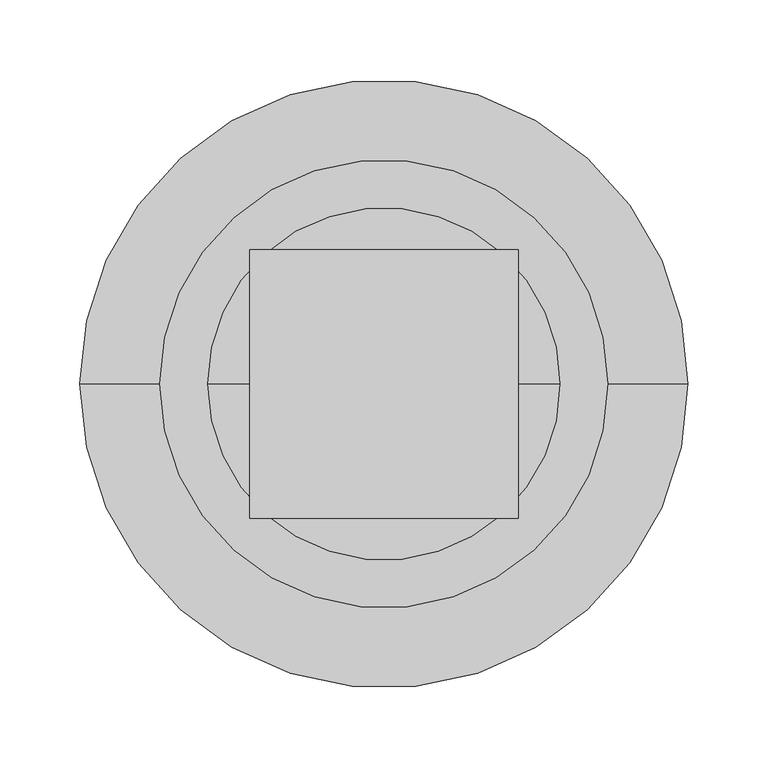
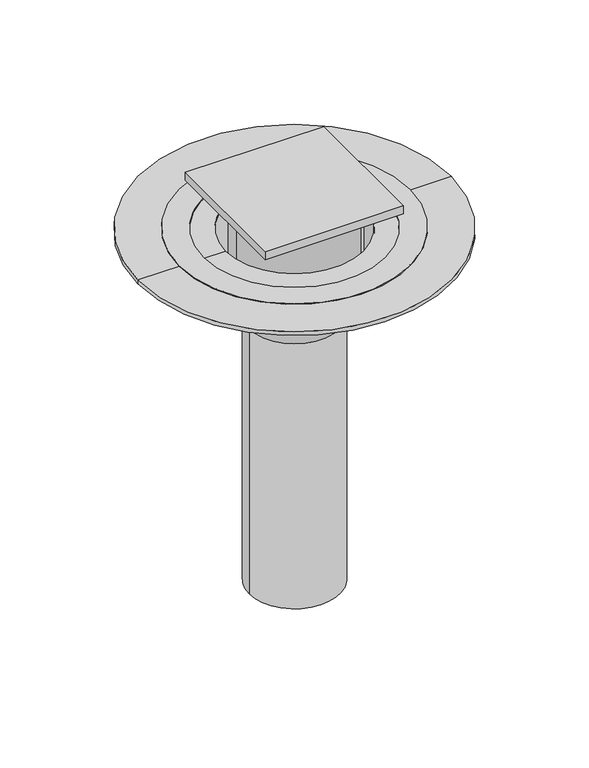
"""IFC4 building model written with IfcOpenShell, lengths in millimetres: proxy geometry, TN_Надставной элемент водоприемной воронки : Надставной элемент с обжимным закручивающемся фланцем, уплотнительным кольцом и трапом для эксплуатируемой кровли."""

from ifc_helpers import new_model, si_unit, point, frame, origin, origin_with_axes, origin_2d, place, context, project, spatial, polyline, circle_curve, trimmed, segment, composite_curve, outline, extrude, source, transform, mapped, element, save
from ifc_brep_helpers import plane_surface, cylinder_surface, revolved_surface, advanced_brep


def specialty_equipment_4cfdb0cb(model_context):
    return source(origin(), model_context, "Body", "SolidModel", [
        extrude(outline(composite_curve([segment(trimmed(circle_curve(origin_2d(), 70.0), [point((-70.0, 0.0))], [point((70.0, 0.0))], False, "CARTESIAN"), True, "CONTINUOUS"), segment(trimmed(circle_curve(origin_2d(), 70.0), [point((70.0, 0.0))], [point((-70.0, 0.0))], False, "CARTESIAN"), True, "CONTINUOUS")], self_intersect=False)), frame((0.0, 0.0, -66.9669914), z_axis=(0.0, 0.0, 1.0), x_axis=(1.0, 0.0, 0.0)), (0.0, 0.0, 1.0), 106.9669914),
        extrude(outline(polyline([(83.890873, 83.890873), (83.890873, -83.890873), (-83.890873, -83.890873), (-83.890873, 83.890873), (83.890873, 83.890873)])), frame((0.0, 0.0, 40.0), z_axis=(0.0, 0.0, 1.0), x_axis=(1.0, 0.0, 0.0)), (0.0, 0.0, 1.0), 10.0),
        extrude(outline(composite_curve([segment(trimmed(circle_curve(origin_2d(), 140.0), [point((-140.0, 0.0))], [point((140.0, 0.0))], False, "CARTESIAN"), True, "CONTINUOUS"), segment(trimmed(circle_curve(origin_2d(), 140.0), [point((140.0, 0.0))], [point((-140.0, 0.0))], False, "CARTESIAN"), True, "CONTINUOUS")], self_intersect=False), holes=[composite_curve([segment(trimmed(circle_curve(origin_2d(), 110.0556416), [point((-110.0556416, 0.0))], [point((110.0556416, 0.0))], True, "CARTESIAN"), True, "CONTINUOUS"), segment(trimmed(circle_curve(origin_2d(), 110.0556416), [point((110.0556416, 0.0))], [point((-110.0556416, 0.0))], True, "CARTESIAN"), True, "CONTINUOUS")], self_intersect=False)]), origin_with_axes(), (0.0, 0.0, 1.0), 1.0),
        advanced_brep(
        [(0.0, 0.0, -450.0), (-55.0, 0.0, -450.0), (55.0, 0.0, -450.0), (190.0, 0.0, 0.0), (-190.0, 0.0, 0.0), (-83.890873, 0.0, 0.0), (83.890873, 0.0, 0.0), (190.0, 0.0, -5.0), (-190.0, 0.0, -5.0), (93.890873, 0.0, -5.0), (-93.890873, 0.0, -5.0), (55.0, 0.0, -110.0), (-55.0, 0.0, -110.0), (-93.890873, 0.0, -71.109127), (93.890873, 0.0, -71.109127), (55.5025253, 0.0, -95.3553391), (-55.5025253, 0.0, -95.3553391), (0.0, 0.0, -95.3553391), (83.890873, 0.0, -66.9669914), (-83.890873, 0.0, -66.9669914)],
        [
            (0, 1),
            (1, 2, circle_curve(frame((0.0, 0.0, -450.0), z_axis=(0.0, 0.0, -1.0), x_axis=(-1.0, 0.0, 0.0)), 55.0)),
            (2, 0),
            (2, 1, circle_curve(frame((0.0, 0.0, -450.0), z_axis=(0.0, 0.0, -1.0), x_axis=(-1.0, 0.0, 0.0)), 55.0)),
            (3, 4, circle_curve(frame((0.0, 0.0, 0.0), z_axis=(0.0, 0.0, 1.0), x_axis=(-1.0, 0.0, 0.0)), 190.0)),
            (4, 5),
            (5, 6, circle_curve(frame((0.0, 0.0, 0.0), z_axis=(0.0, 0.0, -1.0), x_axis=(-1.0, 0.0, 0.0)), 83.890873)),
            (6, 3),
            (4, 3, circle_curve(frame((0.0, 0.0, 0.0), z_axis=(0.0, 0.0, 1.0), x_axis=(-1.0, 0.0, 0.0)), 190.0)),
            (6, 5, circle_curve(frame((0.0, 0.0, 0.0), z_axis=(0.0, 0.0, -1.0), x_axis=(-1.0, 0.0, 0.0)), 83.890873)),
            (7, 8, circle_curve(frame((0.0, 0.0, -5.0), z_axis=(0.0, 0.0, 1.0), x_axis=(-1.0, 0.0, 0.0)), 190.0)),
            (8, 4),
            (3, 7),
            (8, 7, circle_curve(frame((0.0, 0.0, -5.0), z_axis=(0.0, 0.0, 1.0), x_axis=(-1.0, 0.0, 0.0)), 190.0)),
            (9, 10, circle_curve(frame((0.0, 0.0, -5.0), z_axis=(0.0, 0.0, 1.0), x_axis=(-1.0, 0.0, 0.0)), 93.890873)),
            (10, 8),
            (7, 9),
            (10, 9, circle_curve(frame((0.0, 0.0, -5.0), z_axis=(0.0, 0.0, 1.0), x_axis=(-1.0, 0.0, 0.0)), 93.890873)),
            (11, 12, circle_curve(frame((0.0, 0.0, -110.0), z_axis=(0.0, 0.0, 1.0), x_axis=(-1.0, 0.0, 0.0)), 55.0)),
            (12, 13),
            (13, 14, circle_curve(frame((0.0, 0.0, -71.109127), z_axis=(0.0, 0.0, -1.0), x_axis=(-1.0, 0.0, 0.0)), 93.890873)),
            (14, 11),
            (12, 11, circle_curve(frame((0.0, 0.0, -110.0), z_axis=(0.0, 0.0, 1.0), x_axis=(-1.0, 0.0, 0.0)), 55.0)),
            (14, 13, circle_curve(frame((0.0, 0.0, -71.109127), z_axis=(0.0, 0.0, -1.0), x_axis=(-1.0, 0.0, 0.0)), 93.890873)),
            (1, 12),
            (11, 2),
            (13, 10),
            (9, 14),
            (15, 16, circle_curve(frame((0.0, 0.0, -95.3553391), z_axis=(0.0, 0.0, 1.0), x_axis=(-1.0, 0.0, 0.0)), 55.5025253)),
            (16, 17),
            (17, 15),
            (16, 15, circle_curve(frame((0.0, 0.0, -95.3553391), z_axis=(0.0, 0.0, 1.0), x_axis=(-1.0, 0.0, 0.0)), 55.5025253)),
            (18, 19, circle_curve(frame((0.0, 0.0, -66.9669914), z_axis=(0.0, 0.0, 1.0), x_axis=(-1.0, 0.0, 0.0)), 83.890873)),
            (19, 16),
            (15, 18),
            (19, 18, circle_curve(frame((0.0, 0.0, -66.9669914), z_axis=(0.0, 0.0, 1.0), x_axis=(-1.0, 0.0, 0.0)), 83.890873)),
            (5, 19),
            (18, 6),
        ],
        [
            plane_surface(frame((0.0, 0.0, -450.0), z_axis=(0.0, 0.0, -1.0), x_axis=(-1.0, 0.0, 0.0))),
            plane_surface(frame((0.0, 0.0, 0.0), z_axis=(0.0, 0.0, 1.0), x_axis=(-1.0, 0.0, 0.0))),
            cylinder_surface(frame((0.0, 0.0, 0.0), z_axis=(0.0, 0.0, -1.0), x_axis=(-1.0, 0.0, 0.0)), 190.0),
            plane_surface(frame((0.0, 0.0, -5.0), z_axis=(0.0, 0.0, -1.0), x_axis=(-1.0, 0.0, 0.0))),
            revolved_surface(polyline([(-93.890873, 0.0, -71.109127), (-55.0, 0.0, -110.0)]), (0.0, 0.0, 0.0), (0.0, 0.0, -1.0)),
            cylinder_surface(frame((0.0, 0.0, 0.0), z_axis=(0.0, 0.0, -1.0), x_axis=(-1.0, 0.0, 0.0)), 55.0),
            cylinder_surface(frame((0.0, 0.0, 0.0), z_axis=(0.0, 0.0, -1.0), x_axis=(-1.0, 0.0, 0.0)), 93.890873),
            plane_surface(frame((0.0, 0.0, -95.3553391), z_axis=(0.0, 0.0, 1.0), x_axis=(-1.0, 0.0, 0.0))),
            revolved_surface(polyline([(-55.5025253, 0.0, -95.3553391), (-83.890873, 0.0, -66.9669914)]), (0.0, 0.0, 0.0), (0.0, 0.0, -1.0)),
            revolved_surface(polyline([(-83.890873, 0.0, -66.9669914), (-83.890873, 0.0, 0.0)]), (0.0, 0.0, 0.0), (0.0, 0.0, -1.0)),
        ],
        [
            (0, [[1, 2, 3]]),
            (0, [[-3, 4, -1]]),
            (1, [[5, 6, 7, 8]]),
            (1, [[9, -8, 10, -6]]),
            (2, [[11, 12, -5, 13]]),
            (2, [[14, -13, -9, -12]]),
            (3, [[15, 16, -11, 17]]),
            (3, [[18, -17, -14, -16]]),
            (4, [[19, 20, 21, 22]]),
            (4, [[23, -22, 24, -20]]),
            (5, [[-2, 25, -19, 26]]),
            (5, [[-4, -26, -23, -25]]),
            (6, [[-21, 27, -15, 28]]),
            (6, [[-24, -28, -18, -27]]),
            (7, [[29, 30, 31]]),
            (7, [[32, -31, -30]]),
            (8, [[33, 34, -29, 35]]),
            (8, [[36, -35, -32, -34]]),
            (9, [[-7, 37, -33, 38]]),
            (9, [[-10, -38, -36, -37]]),
        ],
    ),
    ])


if __name__ == "__main__":
    model = new_model("IFC4")
    model_context = context("Model", 3, world=origin())
    ifc_project = project(units=[si_unit("LENGTHUNIT", "METRE", prefix="MILLI")], contexts=[model_context])
    site = spatial("IfcSite", under=ifc_project)
    building = spatial("IfcBuilding", under=site)
    placement = place(None, origin())
    specialty_equipment_shape = specialty_equipment_4cfdb0cb(model_context)
    element("IfcBuildingElementProxy", 1, Name="TN_Надставной элемент водоприемной воронки : Надставной элемент с обжимным закручивающемся фланцем, уплотнительным кольцом и трапом для эксплуатируемой кровли", ObjectType="TN_Надставной элемент водоприемной воронки : Надставной элемент с обжимным закручивающемся фланцем, уплотнительным кольцом и трапом для эксплуатируемой кровли", at=placement, inside=building, context=model_context, shape_type="MappedRepresentation", body=[
        mapped(specialty_equipment_shape, transform((0.0, 0.0, 0.0), x_axis=(1.0, 0.0, 0.0), y_axis=(0.0, 1.0, 0.0), z_axis=(0.0, 0.0, 1.0))),
    ])
    save(model, "model.ifc")

# Revit data of these elements
# Type "TN_Надставной элемент водоприемной воронки : Надставной элемент с обжимным закручивающемся фланцем, уплотнительным кольцом и трапом для эксплуатируемой кровли"
#   ADSK_Группирование = "Комплектующие и воронки"
#   Description = "Надставной элемент с обжимным металлическим фланцем и уплотнительным кольцом применяется для создания двух уровневых кровельных воронок. Манжета предотвращает проникновение ливневых стоков в слой теплоизоляции по месту соединения надставного элемента с воронкой. Может быть также использован как самостоятельное изделие подобно воронке с обжимным металлическим фланцем. Также надставной элемент комплектуется уплотнительным кольцом, комплектом гаек и барашков."
#   Manufacturer = "ТехноНИКОЛЬ"
#   URL = "https://shop.tn.ru/nadstavnoj-jelement-s-obzhimnym-zakruchivajuschemsja-flancem-i-uplotnitelnym-kolcom"
#   ADSK_Примечание = ""
#   ADSK_Обозначение = "ТехноНИКОЛЬ"
#   ADSK_Наименование = "Надставной элемент с обжимным закручивающемся  фланцем, уплотнительным кольцом и трапом для эксплуатируемой кровли"
#   ADSK_Марка = ""
#   ADSK_Код изделия = "661129"
#   ADSK_Завод-изготовитель = "ТехноНИКОЛЬ"
#   ADSK_Единица измерения = "шт."
#   ADSK_Группирование = "Комплектующие и воронки"
#   ADSK_URL страницы изделия = "https://shop.tn.ru/nadstavnoj-jelement-s-obzhimnym-zakruchivajuschemsja-flancem-i-uplotnitelnym-kolcom"
#   ADSK_URL документации изделия = "https://shop.tn.ru/media/other_documents/_661129_661126_661128_661127_661133_1.pdf"
#   Тип надставного элемента = 2
#   Радиус = 55 mm
#   Длина расчетная [instance default] = 450 mm
#   Длина отвода [instance default] = 450 mm
#   Высота трапа расчетная [instance default] = 50 mm
#   Высота трапа [instance default] = 50 mm
#   ADSK_Количество = 1
#   Видимость_Листоуловитель [instance default] = no
#   Видимость трапа [instance default] = yes
#   Видимость листоуловителя [instance default] = no
#   Материал_Фланец = TN_Фланец_Красный
#   Материал_Корпус = TN_ПВХ_Черный
#   Default Elevation = 0
# Element 1 (IfcBuildingElementProxy, "TN_Надставной элемент водоприемной воронки : Надставной элемент с обжимным закручивающемся фланцем, уплотнительным кольцом и трапом для эксплуатируемой кровли")
#   Видимость_Листоуловитель = yes
#   Materials on its faces: "TN_ПВХ_Черный", "TN_ПВХ_Серый", "TN_Фланец_Красный"
# Materials
#   "TN_Фланец_Красный": class "Типовые", colour RGB 70 0 0, transparency 0, Cost = 0
#   "TN_ПВХ_Черный": class "Типовые", colour RGB 48 48 48, transparency 0, Cost = 0
#   "TN_ПВХ_Серый": class "Типовые", colour RGB 192 192 192, transparency 0, Cost = 0
